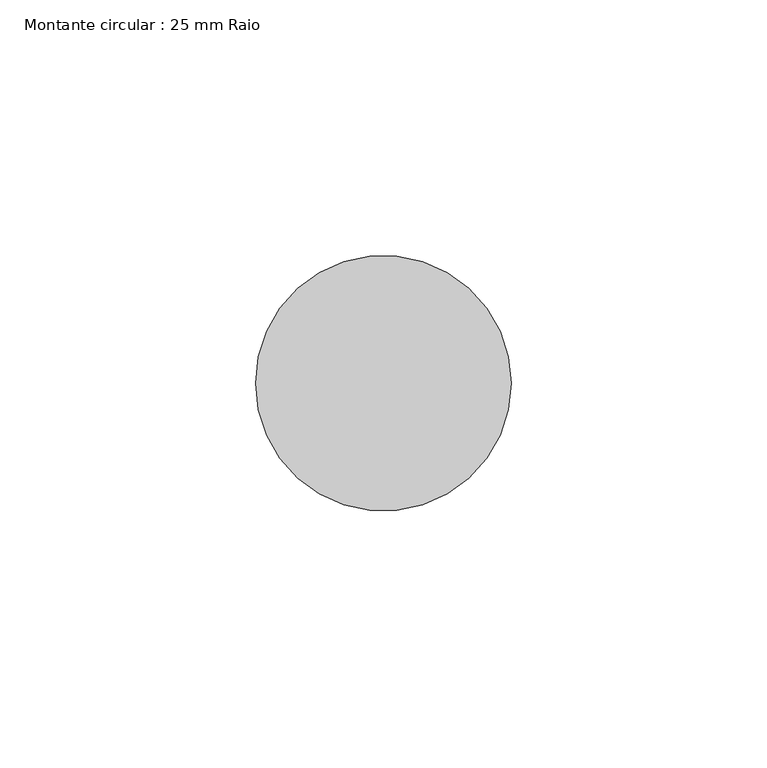
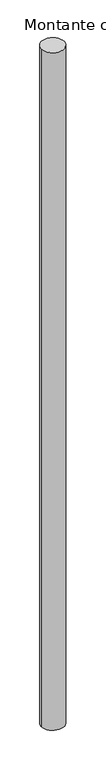
"""IFC4 building model written with IfcOpenShell, lengths in millimetres: member geometry, Montante circular : 25 mm Raio."""

from ifc_helpers import new_model, si_unit, point, frame, origin, origin_2d, place, context, project, spatial, circle_curve, trimmed, segment, composite_curve, outline, extrude, source, transform, mapped, element, save


def montante_circular_25_mm_raio_0f086e2a(model_context):
    return source(origin(), model_context, "Body", "SweptSolid", [
        extrude(outline(composite_curve([segment(trimmed(circle_curve(origin_2d(), 25.0), [point((25.0, 0.0))], [point((-25.0, 0.0))], False, "CARTESIAN"), True, "CONTINUOUS"), segment(trimmed(circle_curve(origin_2d(), 25.0), [point((-25.0, 0.0))], [point((25.0, 0.0))], False, "CARTESIAN"), True, "CONTINUOUS")], self_intersect=False)), frame((0.0, 0.0, -1580.6319563), z_axis=(0.0, 0.0, 1.0), x_axis=(1.0, 0.0, 0.0)), (0.0, 0.0, 1.0), 1580.6319563),
    ])


if __name__ == "__main__":
    model = new_model("IFC4")
    model_context = context("Model", 3, world=origin())
    ifc_project = project(units=[si_unit("LENGTHUNIT", "METRE", prefix="MILLI")], contexts=[model_context])
    site = spatial("IfcSite", under=ifc_project)
    building = spatial("IfcBuilding", under=site)
    placement = place(None, origin())
    montante_circular_25_mm_raio_shape = montante_circular_25_mm_raio_0f086e2a(model_context)
    element("IfcMember", 1, ObjectType="Montante circular : 25 mm Raio", at=placement, inside=building, context=model_context, shape_type="MappedRepresentation", body=[
        mapped(montante_circular_25_mm_raio_shape, transform((0.0, 0.0, 0.0), x_axis=(1.0, 0.0, 0.0), y_axis=(0.0, 1.0, 0.0), z_axis=(0.0, 0.0, 1.0))),
    ])
    save(model, "model.ifc")

# Revit data of these elements
# Type "Montante circular : 25 mm Raio"
#   built-in parameter 1007350 = 0.082021 (stored number, unit not read)
# Element 1 (IfcMember, "Montante circular : 25 mm Raio")
#   Materials on its faces: "Alumín."
# Materials
#   "Alumín.": class "Metal", colour RGB 247 247 247, transparency 0, Description = "Alumín. 6061", Cost = 0
